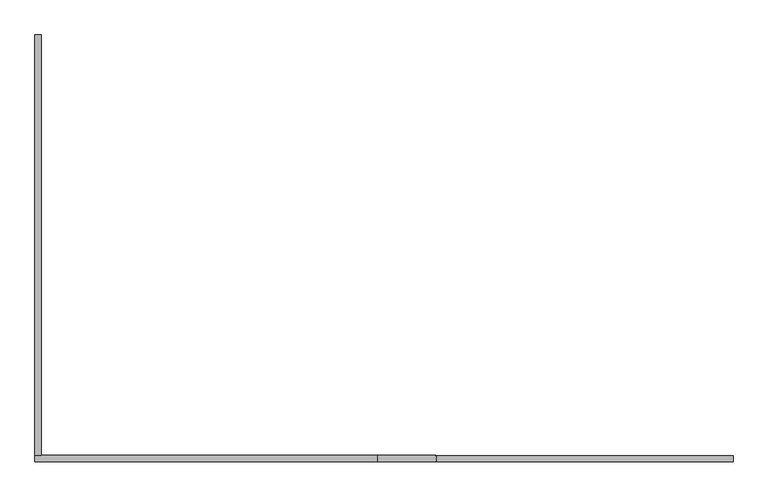
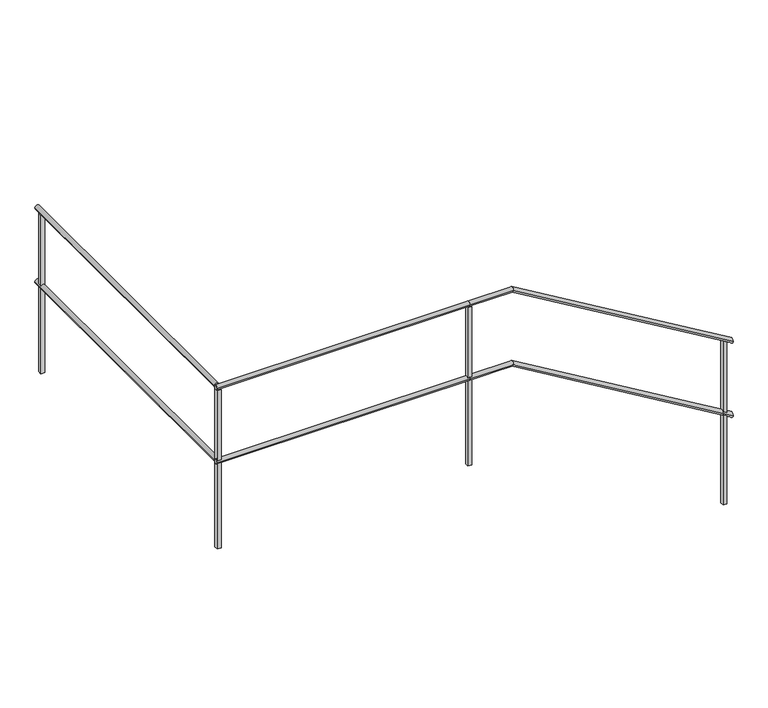
"""IFC4 building model written with IfcOpenShell, lengths in millimetres: railing geometry."""

from ifc_helpers import new_model, si_unit, frame, origin, place, context, project, spatial, polyline, circle_curve, ellipse_curve, outline, extrude, source, transform, mapped, element, save
from ifc_brep_helpers import plane_surface, cylinder_surface, advanced_brep


def railing_8fa59944(model_context):
    return source(origin(), model_context, "Body", "SolidModel", [
        advanced_brep(
        [(26565.4, 649.5208589, 1584.9618634), (26535.4, 649.5208589, 1584.9618634), (26565.4, -1335.0791411, 1584.9618634), (26535.4, -1335.0791411, 1584.9618634)],
        [
            (0, 1, circle_curve(frame((26550.4, 649.5208589, 1584.9618634), z_axis=(0.0, 1.0, 0.0), x_axis=(-1.0, 0.0, 0.0)), 15.0)),
            (1, 0, circle_curve(frame((26550.4, 649.5208589, 1584.9618634), z_axis=(0.0, 1.0, 0.0), x_axis=(-1.0, 0.0, 0.0)), 15.0)),
            (2, 3, circle_curve(frame((26550.4, -1335.0791411, 1584.9618634), z_axis=(0.0, -1.0, 0.0), x_axis=(-1.0, 0.0, 0.0)), 15.0)),
            (3, 2, circle_curve(frame((26550.4, -1335.0791411, 1584.9618634), z_axis=(0.0, -1.0, 0.0), x_axis=(-1.0, 0.0, 0.0)), 15.0)),
            (0, 2),
            (3, 1),
        ],
        [
            plane_surface(frame((26550.4, 649.5208589, 1599.9618634), z_axis=(0.0, 1.0, 0.0), x_axis=(0.0, 0.0, -1.0))),
            plane_surface(frame((26550.4, -1335.0791411, 1599.9618634), z_axis=(0.0, -1.0, 0.0), x_axis=(0.0, 0.0, -1.0))),
            cylinder_surface(frame((26550.4, 649.5208589, 1584.9618634), z_axis=(0.0, 1.0, 0.0), x_axis=(-1.0, 0.0, 0.0)), 15.0),
        ],
        [
            (0, [[1, 2]]),
            (1, [[3, 4]]),
            (2, [[-1, 5, -4, 6]]),
            (2, [[-2, -6, -3, -5]]),
        ],
    ),
        advanced_brep(
        [(26535.4, -1335.0791411, 1584.9618634), (26535.4, -1365.0791411, 1584.9618634), (28150.0, -1335.0791411, 1584.9618634), (28150.0, -1365.0791411, 1584.9618634)],
        [
            (0, 1, circle_curve(frame((26535.4, -1350.0791411, 1584.9618634), z_axis=(-1.0, 0.0, 0.0), x_axis=(0.0, -1.0, 0.0)), 15.0)),
            (1, 0, circle_curve(frame((26535.4, -1350.0791411, 1584.9618634), z_axis=(-1.0, 0.0, 0.0), x_axis=(0.0, -1.0, 0.0)), 15.0)),
            (2, 3, circle_curve(frame((28150.0, -1350.0791411, 1584.9618634), z_axis=(1.0, 0.0, 0.0), x_axis=(0.0, -1.0, 0.0)), 15.0)),
            (3, 2, circle_curve(frame((28150.0, -1350.0791411, 1584.9618634), z_axis=(1.0, 0.0, 0.0), x_axis=(0.0, -1.0, 0.0)), 15.0)),
            (0, 2),
            (3, 1),
        ],
        [
            plane_surface(frame((26535.4, -1350.0791411, 1599.9618634), z_axis=(-1.0, 0.0, 0.0), x_axis=(0.0, 1.0, 0.0))),
            plane_surface(frame((28150.0, -1350.0791411, 1599.9618634), z_axis=(1.0, 0.0, 0.0), x_axis=(0.0, 1.0, 0.0))),
            cylinder_surface(frame((26535.4, -1350.0791411, 1584.9618634), z_axis=(-1.0, 0.0, 0.0), x_axis=(0.0, -1.0, 0.0)), 15.0),
        ],
        [
            (0, [[1, 2]]),
            (1, [[3, 4]]),
            (2, [[-1, 5, -4, 6]]),
            (2, [[-2, -6, -3, -5]]),
        ],
    ),
        advanced_brep(
        [(28150.0, -1335.0791411, 1584.9618634), (28150.0, -1365.0791411, 1584.9618634), (28425.8735614, -1335.0791411, 1584.9618634), (28425.8735614, -1365.0791411, 1584.9618634), (29830.0, -1335.0791411, 749.1723166), (29830.0, -1365.0791411, 749.1723166)],
        [
            (0, 1, circle_curve(frame((28150.0, -1350.0791411, 1584.9618634), z_axis=(-1.0, 0.0, 0.0), x_axis=(0.0, -1.0, 0.0)), 15.0)),
            (1, 0, circle_curve(frame((28150.0, -1350.0791411, 1584.9618634), z_axis=(-1.0, 0.0, 0.0), x_axis=(0.0, -1.0, 0.0)), 15.0)),
            (0, 2),
            (2, 3, ellipse_curve(frame((28425.8735614, -1350.0791411, 1584.9618634), z_axis=(-0.9641817474962142, 0.0, 0.26524245096731175), x_axis=(-0.2652424509673112, 0.0, -0.9641817474962141)), 15.5572329, 15.0)),
            (3, 1),
            (3, 2, ellipse_curve(frame((28425.8735614, -1350.0791411, 1584.9618634), z_axis=(-0.9641817474962142, 0.0, 0.26524245096731175), x_axis=(-0.2652424509673112, 0.0, -0.9641817474962141)), 15.5572329, 15.0)),
            (4, 5, ellipse_curve(frame((29830.0, -1350.0791411, 749.1723166), z_axis=(1.0, 0.0, 0.0), x_axis=(0.0, 0.0, 1.0)), 17.4562134, 15.0)),
            (5, 4, ellipse_curve(frame((29830.0, -1350.0791411, 749.1723166), z_axis=(1.0, 0.0, 0.0), x_axis=(0.0, 0.0, 1.0)), 17.4562134, 15.0)),
            (2, 4),
            (5, 3),
        ],
        [
            plane_surface(frame((28150.0, -1350.0791411, 1599.9618634), z_axis=(-1.0, 0.0, 0.0), x_axis=(0.0, 1.0, 0.0))),
            cylinder_surface(frame((28150.0, -1350.0791411, 1584.9618634), z_axis=(-1.0, 0.0, 0.0), x_axis=(0.0, -1.0, 0.0)), 15.0),
            plane_surface(frame((29830.0, -1350.0791411, 766.62853), z_axis=(1.0, 0.0, 0.0), x_axis=(0.0, 1.0, 0.0))),
            cylinder_surface(frame((28422.3277421, -1350.0791411, 1587.0724701), z_axis=(-0.8592928844097065, 0.0, 0.5114838597676831), x_axis=(0.0, -1.0, 0.0)), 15.0),
        ],
        [
            (0, [[1, 2]]),
            (1, [[-1, 3, 4, 5]]),
            (1, [[-2, -5, 6, -3]]),
            (2, [[7, 8]]),
            (3, [[-4, 9, -8, 10]]),
            (3, [[-6, -10, -7, -9]]),
        ],
    ),
        advanced_brep(
        [(26565.4, 649.5208589, 2084.9618634), (26535.4, 649.5208589, 2084.9618634), (26565.4, -1335.0791411, 2084.9618634), (26535.4, -1335.0791411, 2084.9618634)],
        [
            (0, 1, circle_curve(frame((26550.4, 649.5208589, 2084.9618634), z_axis=(0.0, 1.0, 0.0), x_axis=(-1.0, 0.0, 0.0)), 15.0)),
            (1, 0, circle_curve(frame((26550.4, 649.5208589, 2084.9618634), z_axis=(0.0, 1.0, 0.0), x_axis=(-1.0, 0.0, 0.0)), 15.0)),
            (2, 3, circle_curve(frame((26550.4, -1335.0791411, 2084.9618634), z_axis=(0.0, -1.0, 0.0), x_axis=(-1.0, 0.0, 0.0)), 15.0)),
            (3, 2, circle_curve(frame((26550.4, -1335.0791411, 2084.9618634), z_axis=(0.0, -1.0, 0.0), x_axis=(-1.0, 0.0, 0.0)), 15.0)),
            (0, 2),
            (3, 1),
        ],
        [
            plane_surface(frame((26550.4, 649.5208589, 2099.9618634), z_axis=(0.0, 1.0, 0.0), x_axis=(0.0, 0.0, -1.0))),
            plane_surface(frame((26550.4, -1335.0791411, 2099.9618634), z_axis=(0.0, -1.0, 0.0), x_axis=(0.0, 0.0, -1.0))),
            cylinder_surface(frame((26550.4, 649.5208589, 2084.9618634), z_axis=(0.0, 1.0, 0.0), x_axis=(-1.0, 0.0, 0.0)), 15.0),
        ],
        [
            (0, [[1, 2]]),
            (1, [[3, 4]]),
            (2, [[-1, 5, -4, 6]]),
            (2, [[-2, -6, -3, -5]]),
        ],
    ),
        advanced_brep(
        [(26535.4, -1335.0791411, 2084.9618634), (26535.4, -1365.0791411, 2084.9618634), (28150.0, -1335.0791411, 2084.9618634), (28150.0, -1365.0791411, 2084.9618634)],
        [
            (0, 1, circle_curve(frame((26535.4, -1350.0791411, 2084.9618634), z_axis=(-1.0, 0.0, 0.0), x_axis=(0.0, -1.0, 0.0)), 15.0)),
            (1, 0, circle_curve(frame((26535.4, -1350.0791411, 2084.9618634), z_axis=(-1.0, 0.0, 0.0), x_axis=(0.0, -1.0, 0.0)), 15.0)),
            (2, 3, circle_curve(frame((28150.0, -1350.0791411, 2084.9618634), z_axis=(1.0, 0.0, 0.0), x_axis=(0.0, -1.0, 0.0)), 15.0)),
            (3, 2, circle_curve(frame((28150.0, -1350.0791411, 2084.9618634), z_axis=(1.0, 0.0, 0.0), x_axis=(0.0, -1.0, 0.0)), 15.0)),
            (0, 2),
            (3, 1),
        ],
        [
            plane_surface(frame((26535.4, -1350.0791411, 2099.9618634), z_axis=(-1.0, 0.0, 0.0), x_axis=(0.0, 1.0, 0.0))),
            plane_surface(frame((28150.0, -1350.0791411, 2099.9618634), z_axis=(1.0, 0.0, 0.0), x_axis=(0.0, 1.0, 0.0))),
            cylinder_surface(frame((26535.4, -1350.0791411, 2084.9618634), z_axis=(-1.0, 0.0, 0.0), x_axis=(0.0, -1.0, 0.0)), 15.0),
        ],
        [
            (0, [[1, 2]]),
            (1, [[3, 4]]),
            (2, [[-1, 5, -4, 6]]),
            (2, [[-2, -6, -3, -5]]),
        ],
    ),
        advanced_brep(
        [(28150.0, -1335.0791411, 2084.9618634), (28150.0, -1365.0791411, 2084.9618634), (28425.8735614, -1335.0791411, 2084.9618634), (28425.8735614, -1365.0791411, 2084.9618634), (29830.0, -1335.0791411, 1249.1723166), (29830.0, -1365.0791411, 1249.1723166)],
        [
            (0, 1, circle_curve(frame((28150.0, -1350.0791411, 2084.9618634), z_axis=(-1.0, 0.0, 0.0), x_axis=(0.0, -1.0, 0.0)), 15.0)),
            (1, 0, circle_curve(frame((28150.0, -1350.0791411, 2084.9618634), z_axis=(-1.0, 0.0, 0.0), x_axis=(0.0, -1.0, 0.0)), 15.0)),
            (0, 2),
            (2, 3, ellipse_curve(frame((28425.8735614, -1350.0791411, 2084.9618634), z_axis=(-0.9641817474962142, 0.0, 0.26524245096731175), x_axis=(-0.2652424509673112, 0.0, -0.9641817474962141)), 15.5572329, 15.0)),
            (3, 1),
            (3, 2, ellipse_curve(frame((28425.8735614, -1350.0791411, 2084.9618634), z_axis=(-0.9641817474962142, 0.0, 0.26524245096731175), x_axis=(-0.2652424509673112, 0.0, -0.9641817474962141)), 15.5572329, 15.0)),
            (4, 5, ellipse_curve(frame((29830.0, -1350.0791411, 1249.1723166), z_axis=(1.0, 0.0, 0.0), x_axis=(0.0, 0.0, 1.0)), 17.4562134, 15.0)),
            (5, 4, ellipse_curve(frame((29830.0, -1350.0791411, 1249.1723166), z_axis=(1.0, 0.0, 0.0), x_axis=(0.0, 0.0, 1.0)), 17.4562134, 15.0)),
            (2, 4),
            (5, 3),
        ],
        [
            plane_surface(frame((28150.0, -1350.0791411, 2099.9618634), z_axis=(-1.0, 0.0, 0.0), x_axis=(0.0, 1.0, 0.0))),
            cylinder_surface(frame((28150.0, -1350.0791411, 2084.9618634), z_axis=(-1.0, 0.0, 0.0), x_axis=(0.0, -1.0, 0.0)), 15.0),
            plane_surface(frame((29830.0, -1350.0791411, 1266.62853), z_axis=(1.0, 0.0, 0.0), x_axis=(0.0, 1.0, 0.0))),
            cylinder_surface(frame((28422.3277421, -1350.0791411, 2087.0724701), z_axis=(-0.8592928844097065, 0.0, 0.5114838597676831), x_axis=(0.0, -1.0, 0.0)), 15.0),
        ],
        [
            (0, [[1, 2]]),
            (1, [[-1, 3, 4, 5]]),
            (1, [[-2, -5, 6, -3]]),
            (2, [[7, 8]]),
            (3, [[-4, 9, -8, 10]]),
            (3, [[-6, -10, -7, -9]]),
        ],
    ),
        extrude(outline(polyline([(28137.5, -1362.5791411), (28137.5, -1337.5791411), (28162.5, -1337.5791411), (28162.5, -1362.5791411), (28137.5, -1362.5791411)])), frame((0.0, 0.0, 999.9618634), z_axis=(0.0, 0.0, 1.0), x_axis=(1.0, 0.0, 0.0)), (0.0, 0.0, 1.0), 1070.0),
        extrude(outline(polyline([(26537.9, -1337.5791411), (26562.9, -1337.5791411), (26562.9, -1362.5791411), (26537.9, -1362.5791411), (26537.9, -1337.5791411)])), frame((0.0, 0.0, 999.9618634), z_axis=(0.0, 0.0, 1.0), x_axis=(1.0, 0.0, 0.0)), (0.0, 0.0, 1.0), 1070.0),
        extrude(outline(polyline([(1273.830911, 29767.5), (166.62853, 29767.5), (166.62853, 29792.5), (1258.9499586, 29792.5), (1273.830911, 29767.5)])), frame((0.0, -1362.5791411, 0.0), z_axis=(0.0, 1.0, 0.0), x_axis=(0.0, 0.0, 1.0)), (0.0, 0.0, 1.0), 25.0),
        extrude(outline(polyline([(26537.9, 612.0208589), (26562.9, 612.0208589), (26562.9, 587.0208589), (26537.9, 587.0208589), (26537.9, 612.0208589)])), frame((0.0, 0.0, 999.9618634), z_axis=(0.0, 0.0, 1.0), x_axis=(1.0, 0.0, 0.0)), (0.0, 0.0, 1.0), 1070.0),
    ])


if __name__ == "__main__":
    model = new_model("IFC4")
    model_context = context("Model", 3, world=origin())
    ifc_project = project(units=[si_unit("LENGTHUNIT", "METRE", prefix="MILLI")], contexts=[model_context])
    site = spatial("IfcSite", under=ifc_project)
    building = spatial("IfcBuilding", under=site)
    placement = place(None, origin())
    railing_shape = railing_8fa59944(model_context)
    element("IfcRailing", 1, at=placement, inside=building, context=model_context, shape_type="MappedRepresentation", body=[
        mapped(railing_shape, transform((0.0, 0.0, 0.0), x_axis=(1.0, 0.0, 0.0), y_axis=(0.0, 1.0, 0.0), z_axis=(0.0, 0.0, 1.0))),
    ])
    save(model, "model.ifc")
